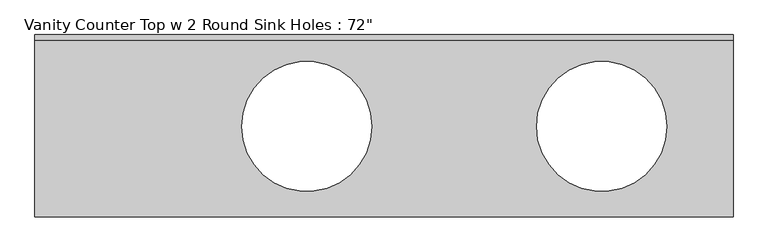
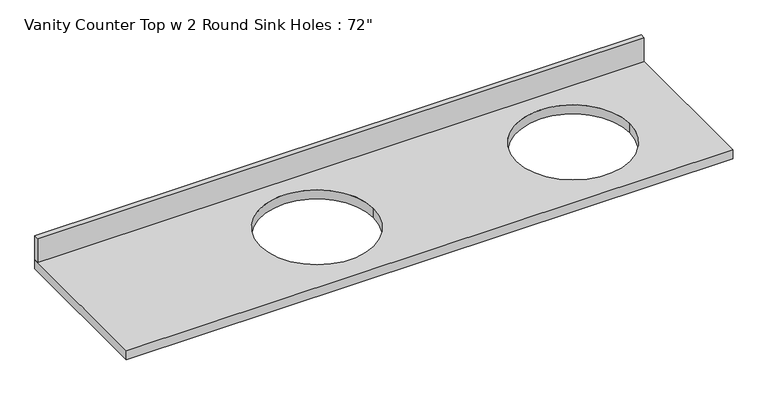
"""IFC4 building model written with IfcOpenShell, lengths in millimetres: furniture geometry."""

from ifc_helpers import new_model, si_unit, point, frame, frame_2d, origin, place, context, project, spatial, polyline, circle_curve, trimmed, segment, composite_curve, outline, extrude, source, transform, mapped, element, save


def furniture_9fbd7df7(model_context):
    return source(origin(), model_context, "Body", "SweptSolid", [
        extrude(outline(polyline([(-1327.4622951, 0.0), (1102.6033299, 0.0), (1102.6033299, -19.05), (-1327.4622951, -19.05), (-1327.4622951, 0.0)])), frame((0.0, 0.0, 787.4), z_axis=(0.0, 0.0, 1.0), x_axis=(1.0, 0.0, 0.0)), (0.0, 0.0, 1.0), 101.6),
        extrude(outline(polyline([(1102.6033299, 0.0), (1102.6033299, -635.0), (-1327.4622951, -635.0), (-1327.4622951, 0.0), (1102.6033299, 0.0)]), holes=[composite_curve([segment(trimmed(circle_curve(frame_2d((-381.3122951, -319.285285)), 226.814715), [point((-608.1270101, -319.285285))], [point((-154.4975801, -319.285285))], True, "CARTESIAN"), True, "CONTINUOUS"), segment(trimmed(circle_curve(frame_2d((-381.3122951, -319.285285)), 226.814715), [point((-154.4975801, -319.285285))], [point((-608.1270101, -319.285285))], True, "CARTESIAN"), True, "CONTINUOUS")], self_intersect=False), composite_curve([segment(trimmed(circle_curve(frame_2d((645.4033299, -319.285285)), 226.814715), [point((418.5886149, -319.285285))], [point((872.2180449, -319.285285))], True, "CARTESIAN"), True, "CONTINUOUS"), segment(trimmed(circle_curve(frame_2d((645.4033299, -319.285285)), 226.814715), [point((872.2180449, -319.285285))], [point((418.5886149, -319.285285))], True, "CARTESIAN"), True, "CONTINUOUS")], self_intersect=False)]), frame((0.0, 0.0, 749.3), z_axis=(0.0, 0.0, 1.0), x_axis=(1.0, 0.0, 0.0)), (0.0, 0.0, 1.0), 38.1),
    ])


if __name__ == "__main__":
    model = new_model("IFC4")
    model_context = context("Model", 3, world=origin())
    ifc_project = project(units=[si_unit("LENGTHUNIT", "METRE", prefix="MILLI")], contexts=[model_context])
    site = spatial("IfcSite", under=ifc_project)
    building = spatial("IfcBuilding", under=site)
    placement = place(None, origin())
    furniture_shape = furniture_9fbd7df7(model_context)
    element("IfcFurniture", 1, ObjectType="Vanity Counter Top w 2 Round Sink Holes : 72\"", at=placement, inside=building, context=model_context, shape_type="MappedRepresentation", body=[
        mapped(furniture_shape, transform((0.0, 0.0, 0.0), x_axis=(1.0, 0.0, 0.0), y_axis=(0.0, 1.0, 0.0), z_axis=(0.0, 0.0, 1.0))),
    ])
    save(model, "model.ifc")

# Revit data of these elements
# Type "Vanity Counter Top w 2 Round Sink Holes : 72\""
#   Assembly Code = "C1030400"
#   Sink Location Right = 1' - 6"
#   Counter Thickness = 0' - 1 1/2"
#   Depth = 2' - 1"
#   Height = 2' - 7"
#   Length [instance default] = 6' - 0"
#   Sink Location Left [instance default] = 1' - 6"
#   Sink Location To Wall [instance default] = 0' - 4"
#   Sink Opening Width [instance default] = 1' - 5"
#   Counter Top = Counter Top
# Element 1 (IfcFurniture, "Vanity Counter Top w 2 Round Sink Holes : 72\"")
#   Length = 7' - 11 43/64"
#   Sink Location Left = 3' - 1 1/4"
#   Sink Location To Wall = 0' - 4.14057"
#   Sink Opening Width = 1' - 4.85943"
#   Materials on its faces: "Counter Top"
# Materials
#   "Counter Top": class "Wood", colour RGB 226 177 128, transparency 0
